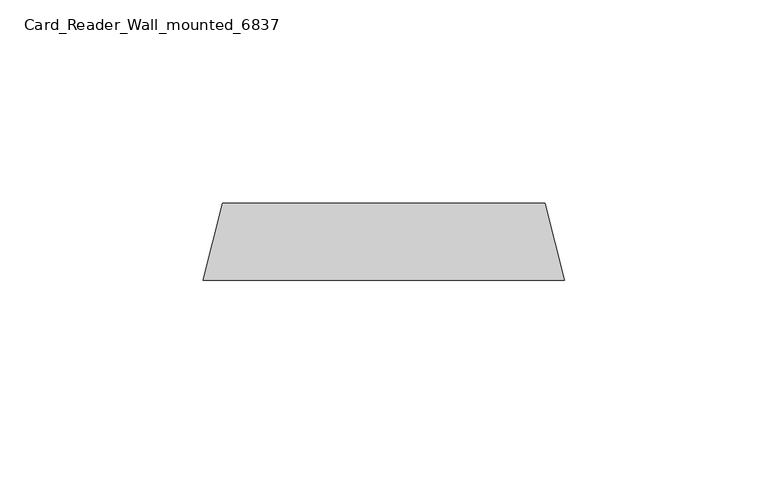
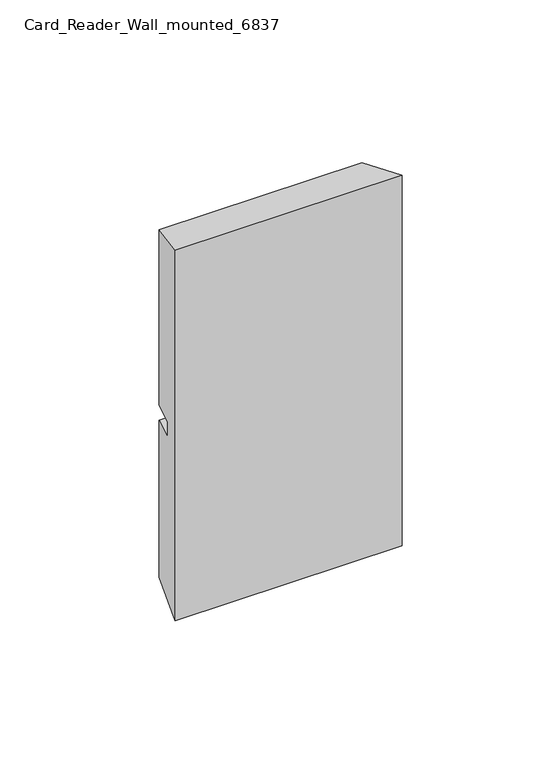
"""IFC4 building model written with IfcOpenShell, lengths in millimetres: proxy geometry, Card_Reader_Wall_mounted_6837 : swipe."""

from ifc_helpers import new_model, si_unit, origin, place, context, project, spatial, faceted_brep, source, transform, mapped, element, save


def card_reader_wall_mounted_6837_e02ab20a(model_context):
    return source(origin(), model_context, "Body", "Brep", [
        faceted_brep([(20.6375, 106.4392764, 1265.2375), (100.0125, 106.4392764, 1265.2375), (100.0125, 106.4392764, 1192.6911313), (20.6375, 106.4392764, 1192.6911313), (100.0125, 106.4392764, 1121.2536313), (20.6375, 106.4392764, 1121.2536313), (20.6375, 106.4392764, 1186.3411313), (100.0125, 106.4392764, 1186.3411313), (15.875, 87.5, 1270.0), (15.875, 87.5, 1116.4911313), (104.775, 87.5, 1116.4911313), (104.775, 87.5, 1270.0), (102.4977808, 96.5559335, 1186.3411313), (102.4977808, 96.5559335, 1192.6911313), (18.1522192, 96.5559335, 1192.6911313), (18.1522192, 96.5559335, 1186.3411313)], [[[0, 1, 2, 3]], [[4, 5, 6, 7]], [[8, 9, 10, 11]], [[1, 0, 8, 11]], [[11, 10, 4, 7, 12, 13, 2, 1]], [[5, 4, 10, 9]], [[9, 8, 0, 3, 14, 15, 6, 5]], [[14, 13, 12, 15]], [[15, 12, 7, 6]], [[13, 14, 3, 2]]]),
    ])


if __name__ == "__main__":
    model = new_model("IFC4")
    model_context = context("Model", 3, world=origin())
    ifc_project = project(units=[si_unit("LENGTHUNIT", "METRE", prefix="MILLI")], contexts=[model_context])
    site = spatial("IfcSite", under=ifc_project)
    building = spatial("IfcBuilding", under=site)
    placement = place(None, origin())
    card_reader_wall_mounted_6837_shape = card_reader_wall_mounted_6837_e02ab20a(model_context)
    element("IfcBuildingElementProxy", 1, Name="Card_Reader_Wall_mounted_6837 : swipe", ObjectType="Card_Reader_Wall_mounted_6837 : swipe", at=placement, inside=building, context=model_context, shape_type="MappedRepresentation", body=[
        mapped(card_reader_wall_mounted_6837_shape, transform((0.0, 0.0, 0.0), x_axis=(1.0, 0.0, 0.0), y_axis=(0.0, 1.0, 0.0), z_axis=(0.0, 0.0, 1.0))),
    ])
    save(model, "model.ifc")

# Revit data of these elements
# Type "Card_Reader_Wall_mounted_6837 : swipe"
#   COBie.Type.CreatedBy = "design@eagle.com"
#   COBie.Type.CreatedOn = "2016-09-13T05:47:35"
#   COBie.Type.Name = "Security Devices_Card_Reader_Wall_mounted_6837_swipe"
#   COBie.Type.Category = "23-85 30 11 : Access Controls"
#   COBie.Type.Description = ""
#   COBie.Type.Manufacturer = ""
#   COBie.Type.ModelNumber = ""
#   COBie.Type.ReplacementCost = 0
#   Width = 69.85 mm
#   Placement Height = 304.8 mm
#   Height = 114.3 mm
#   COBie.Type = yes
#   Material = Plastic - Black
#   Assembly Code = ""
# Element 1 (IfcBuildingElementProxy, "Card_Reader_Wall_mounted_6837 : swipe")
#   Materials on its faces: "Plastic - Black"
# Materials
#   "Plastic - Black": class "Plastic", colour RGB 0 0 0, transparency 0
